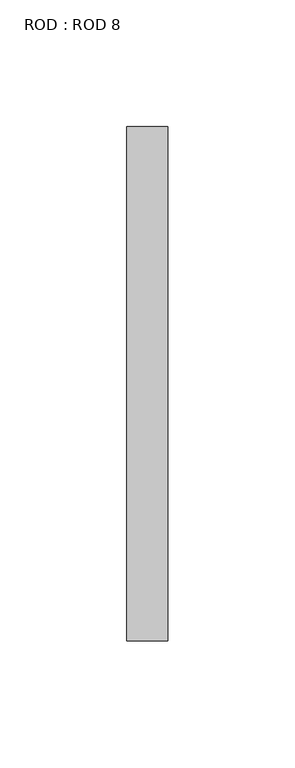
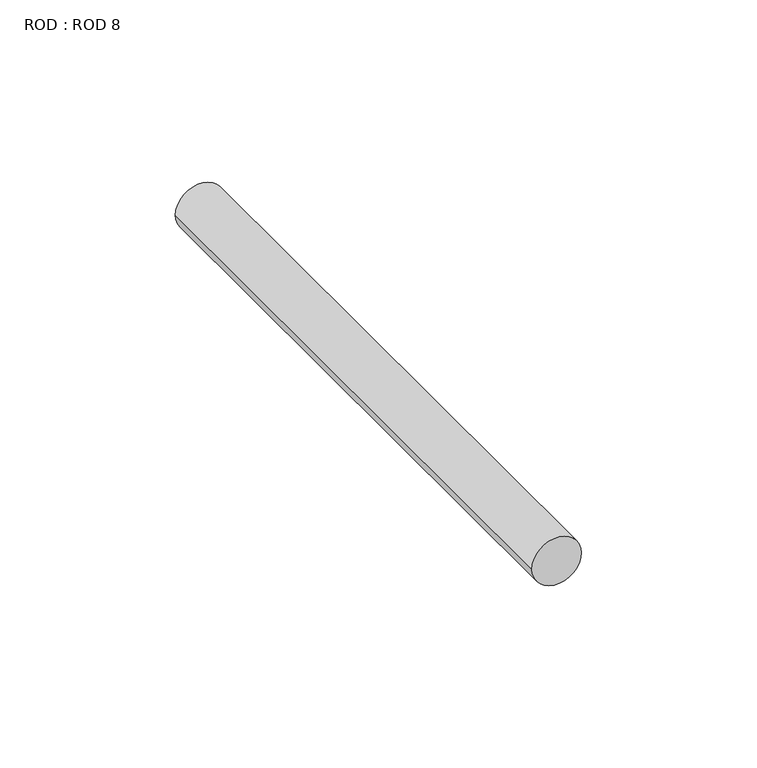
"""IFC4 building model written with IfcOpenShell, lengths in millimetres: proxy geometry, ROD : ROD 8."""

from ifc_helpers import new_model, si_unit, point, frame, origin, origin_2d, place, context, project, spatial, circle_curve, trimmed, segment, composite_curve, outline, extrude, source, transform, mapped, element, save


def rod_rod_8_5da43aea(model_context):
    return source(origin(), model_context, "Body", "SweptSolid", [
        extrude(outline(composite_curve([segment(trimmed(circle_curve(origin_2d(), 8.1359375), [point((0.0, 8.1359375))], [point((0.0, -8.1359375))], False, "CARTESIAN"), True, "CONTINUOUS"), segment(trimmed(circle_curve(origin_2d(), 8.1359375), [point((0.0, -8.1359375))], [point((0.0, 8.1359375))], False, "CARTESIAN"), True, "CONTINUOUS")], self_intersect=False)), frame((0.0, -152.4, 0.0), z_axis=(0.0, 1.0, 0.0), x_axis=(0.0, 0.0, 1.0)), (0.0, 0.0, 1.0), 203.2),
    ])


if __name__ == "__main__":
    model = new_model("IFC4")
    model_context = context("Model", 3, world=origin())
    ifc_project = project(units=[si_unit("LENGTHUNIT", "METRE", prefix="MILLI")], contexts=[model_context])
    site = spatial("IfcSite", under=ifc_project)
    building = spatial("IfcBuilding", under=site)
    placement = place(None, origin())
    rod_rod_8_shape = rod_rod_8_5da43aea(model_context)
    element("IfcBuildingElementProxy", 1, Name="ROD : ROD 8", ObjectType="ROD : ROD 8", at=placement, inside=building, context=model_context, shape_type="MappedRepresentation", body=[
        mapped(rod_rod_8_shape, transform((0.0, 0.0, 0.0), x_axis=(1.0, 0.0, 0.0), y_axis=(0.0, 1.0, 0.0), z_axis=(0.0, 0.0, 1.0))),
    ])
    save(model, "model.ifc")

# Revit data of these elements
# Type "ROD : ROD 8"
#   lenght = 0' - 8"
#   Radius = 0' - 0 41/128"
#   material [instance default] = 3/4" GALV. THRU BOLTS
# Materials
#   "3/4\" GALV. THRU BOLTS": class "Generic", colour RGB 105 69 171, transparency 0, Cost = 0
